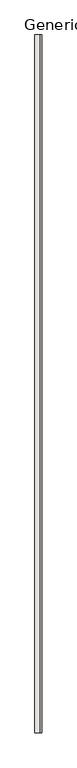
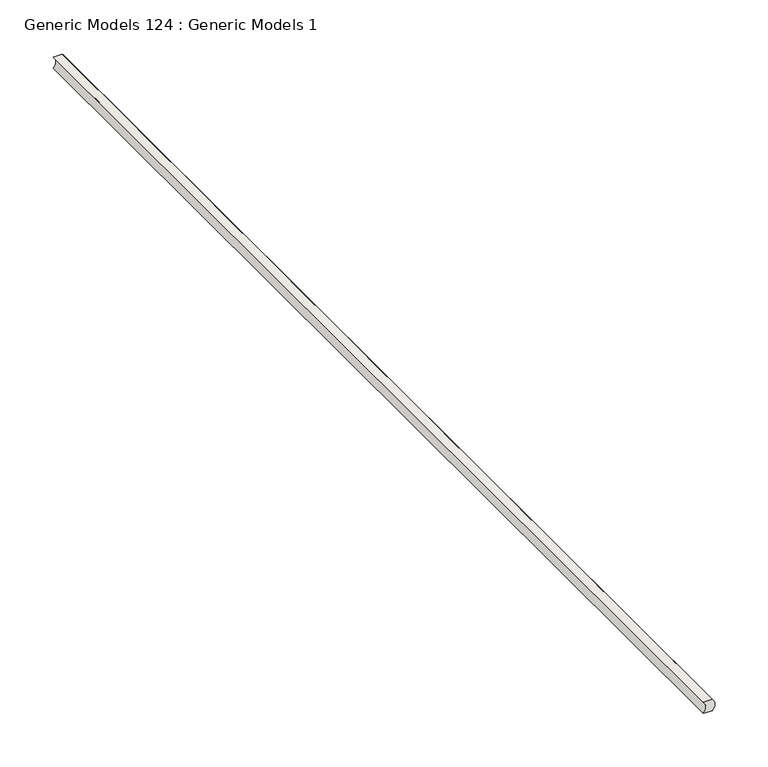
"""IFC4 building model written with IfcOpenShell, lengths in millimetres: wall geometry, Generic Models 124 : Generic Models 1."""

import ifcopenshell
import ifcopenshell.guid

model = None  # the IFC model being written
_history = None  # IfcOwnerHistory: only IFC2X3 demands one
_inside = {}  # id of a spatial element -> (the spatial element, [elements in it])
_under = {}  # id of a project, library or spatial element -> (it, [spatial elements below it])
_declared = {}  # id of a project -> (the project, [libraries it declares])
_typed = {}  # id of a type object -> (the type object, [elements of that type])
_made_of = {}  # id of a material, layer set ... -> (it, [elements and type objects made of it])


def new_model(schema):
    """Start an empty IFC model of exactly this schema.

    Asked for "IFC4X3", IfcOpenShell would pick the latest addendum, in which some entities
    have other attributes; the version numbers below select the first issue.
    IFC2X3 requires an IfcOwnerHistory on every rooted entity: one is made here for all.
    """
    global model, _history
    if schema == "IFC4X3":
        model = ifcopenshell.file(schema_version=(4, 3, 0, 0))
    else:
        model = ifcopenshell.file(schema=schema)
    _inside.clear()
    _under.clear()
    _declared.clear()
    _typed.clear()
    _made_of.clear()
    _history = None
    if model.schema == "IFC2X3":
        org = make("IfcOrganization", Name="unknown")
        user = make(
            "IfcPersonAndOrganization",
            ThePerson=make("IfcPerson", FamilyName="unknown"),
            TheOrganization=org,
        )
        app = make(
            "IfcApplication",
            ApplicationDeveloper=org,
            Version="unknown",
            ApplicationFullName="unknown",
            ApplicationIdentifier="unknown",
        )
        _history = make(
            "IfcOwnerHistory",
            OwningUser=user,
            OwningApplication=app,
            ChangeAction="ADDED",
            CreationDate=0,
        )
    return model


def make(cls, **values):
    """One entity of the class cls with the attributes given. An attribute that is None is left unset."""
    return model.create_entity(
        cls, **{name: value for name, value in values.items() if value is not None}
    )


def rooted(cls, **values):
    """An entity with a GlobalId (a new one), such as an element, a storey or a relation."""
    return make(cls, GlobalId=ifcopenshell.guid.new(), OwnerHistory=_history, **values)


def si_unit(unit_type, name, prefix=None):
    """IfcSIUnit, for example si_unit("LENGTHUNIT", "METRE", prefix="MILLI")."""
    return make("IfcSIUnit", UnitType=unit_type, Prefix=prefix, Name=name)


def assignment(units):
    """IfcUnitAssignment: the units of a project."""
    return None if units is None else make("IfcUnitAssignment", Units=units)


def point(xyz):
    """IfcCartesianPoint."""
    return None if xyz is None else make("IfcCartesianPoint", Coordinates=xyz)


def direction(xyz):
    """IfcDirection."""
    return None if xyz is None else make("IfcDirection", DirectionRatios=xyz)


def frame(location, z_axis=None, x_axis=None):
    """IfcAxis2Placement3D, a coordinate frame: its origin and axes. An axis left out is left unset."""
    return make(
        "IfcAxis2Placement3D",
        Location=point(location),
        Axis=direction(z_axis),
        RefDirection=direction(x_axis),
    )


def frame_2d(location, x_axis=None):
    """IfcAxis2Placement2D, a coordinate frame in the plane: its origin and x axis."""
    return make(
        "IfcAxis2Placement2D", Location=point(location), RefDirection=direction(x_axis)
    )


def origin():
    """The frame at (0, 0, 0) with its axes left unset."""
    return frame((0.0, 0.0, 0.0))


def place(relative_to, where):
    """IfcLocalPlacement: puts the frame where relative to a parent placement (None: the world)."""
    return make(
        "IfcLocalPlacement", PlacementRelTo=relative_to, RelativePlacement=where
    )


def context(
    kind, dimensions, precision=None, world=None, true_north=None, identifier=None
):
    """IfcGeometricRepresentationContext, for example the 3D "Model" context."""
    return make(
        "IfcGeometricRepresentationContext",
        ContextIdentifier=identifier,
        ContextType=kind,
        CoordinateSpaceDimension=dimensions,
        Precision=precision,
        WorldCoordinateSystem=world,
        TrueNorth=true_north,
    )


def project(units=None, contexts=None):
    """IfcProject with its units and contexts."""
    return rooted(
        "IfcProject",
        Name="project",
        RepresentationContexts=contexts,
        UnitsInContext=assignment(units),
    )


def spatial(cls, under=None, at=None, **own):
    """A site, building, storey or space (cls), placed at a placement, below another one or the project."""
    s = rooted(cls, ObjectPlacement=at, **own)
    if under is not None:
        _under.setdefault(under.id(), (under, []))[1].append(s)
    return s


def polyline(points):
    """IfcPolyline through the points."""
    return make("IfcPolyline", Points=[point(p) for p in points])


def circle_curve(where, radius):
    """IfcCircle in the frame where."""
    return make("IfcCircle", Position=where, Radius=radius)


def trimmed(basis, trim1, trim2, sense, master):
    """IfcTrimmedCurve: the piece of a basis curve between two trims."""
    return make(
        "IfcTrimmedCurve",
        BasisCurve=basis,
        Trim1=trim1,
        Trim2=trim2,
        SenseAgreement=sense,
        MasterRepresentation=master,
    )


def segment(curve, same_sense, transition):
    """IfcCompositeCurveSegment."""
    return make(
        "IfcCompositeCurveSegment",
        Transition=transition,
        SameSense=same_sense,
        ParentCurve=curve,
    )


def composite_curve(segments, self_intersect=None):
    """IfcCompositeCurve: segments joined end to end."""
    return make("IfcCompositeCurve", Segments=segments, SelfIntersect=self_intersect)


def outline(outer, holes=None, kind="AREA"):
    """IfcArbitraryClosedProfileDef: a profile drawn as a closed curve; with holes, ...WithVoids."""
    if holes is None:
        return make("IfcArbitraryClosedProfileDef", ProfileType=kind, OuterCurve=outer)
    return make(
        "IfcArbitraryProfileDefWithVoids",
        ProfileType=kind,
        OuterCurve=outer,
        InnerCurves=holes,
    )


def extrude(swept, where, along, depth):
    """IfcExtrudedAreaSolid: the profile swept, set in the frame where, extruded along a direction by depth."""
    return make(
        "IfcExtrudedAreaSolid",
        SweptArea=swept,
        Position=where,
        ExtrudedDirection=direction(along),
        Depth=depth,
    )


def shape(context_of_items, identifier, shape_type, items):
    """IfcShapeRepresentation: the items that make up one representation, for example the "Body"."""
    return make(
        "IfcShapeRepresentation",
        ContextOfItems=context_of_items,
        RepresentationIdentifier=identifier,
        RepresentationType=shape_type,
        Items=items,
    )


def source(mapping_origin, context_of_items, identifier, shape_type, items):
    """IfcRepresentationMap: a shape defined once, which mapped items show again and again."""
    return make(
        "IfcRepresentationMap",
        MappingOrigin=mapping_origin,
        MappedRepresentation=shape(context_of_items, identifier, shape_type, items),
    )


def transform(
    local_origin,
    x_axis=None,
    y_axis=None,
    z_axis=None,
    scale=None,
    scale2=None,
    scale3=None,
    uniform=True,
):
    """IfcCartesianTransformationOperator3D, or its non-uniform kind. x_axis, y_axis, z_axis: its Axis1, 2, 3."""
    if uniform:
        return make(
            "IfcCartesianTransformationOperator3D",
            Axis1=direction(x_axis),
            Axis2=direction(y_axis),
            LocalOrigin=point(local_origin),
            Scale=scale,
            Axis3=direction(z_axis),
        )
    return make(
        "IfcCartesianTransformationOperator3DnonUniform",
        Axis1=direction(x_axis),
        Axis2=direction(y_axis),
        LocalOrigin=point(local_origin),
        Scale=scale,
        Axis3=direction(z_axis),
        Scale2=scale2,
        Scale3=scale3,
    )


def mapped(mapping_source, mapping_target):
    """IfcMappedItem: shows the shape of a source again, moved by a transform."""
    return make(
        "IfcMappedItem", MappingSource=mapping_source, MappingTarget=mapping_target
    )


def made_of(thing, what):
    """Note that an element or type object is made of a material, layer set ...; save() writes the relation."""
    if what is not None:
        _made_of.setdefault(what.id(), (what, []))[1].append(thing)
    return thing


def element(
    cls,
    number,
    at=None,
    inside=None,
    cuts=None,
    type_object=None,
    material=None,
    context=None,
    identifier="Body",
    shape_type=None,
    held_by="IfcProductDefinitionShape",
    body=None,
    shapes=None,
    **own,
):
    """One element of the class cls, such as IfcWall. Its Tag is "e" and its number.

    at: its placement. inside: the storey or other place that contains it. cuts: it is an
    opening in that element (IfcRelVoidsElement). A single representation is given by context,
    identifier, shape_type and body (its items); several are given by shapes. held_by: the class
    of the entity that holds the representations. save() writes the other relations.
    """
    e = rooted(cls, Tag="e%d" % number, ObjectPlacement=at, **own)
    if body is not None:
        shapes = [shape(context, identifier, shape_type, body)]
    if shapes is not None:
        e.Representation = make(held_by, Representations=shapes)
    if inside is not None:
        _inside.setdefault(inside.id(), (inside, []))[1].append(e)
    if cuts is not None:
        rooted(
            "IfcRelVoidsElement", RelatingBuildingElement=cuts, RelatedOpeningElement=e
        )
    if type_object is not None:
        _typed.setdefault(type_object.id(), (type_object, []))[1].append(e)
    return made_of(e, material)


def aggregate(whole, parts):
    """IfcRelAggregates: a whole, such as a stair, and the parts it consists of."""
    return rooted("IfcRelAggregates", RelatingObject=whole, RelatedObjects=parts)


def save(model, path):
    """Write the relations noted so far, then the file.

    IfcRelAggregates (storeys below a building ...), IfcRelContainedInSpatialStructure (elements
    in a storey), IfcRelDefinesByType, IfcRelAssociatesMaterial and IfcRelDeclares: one each for
    every whole, place, type object, material and project.
    """
    for whole, parts in _under.values():
        aggregate(whole, parts)
    for where, things in _inside.values():
        rooted(
            "IfcRelContainedInSpatialStructure",
            RelatedElements=things,
            RelatingStructure=where,
        )
    for kind, things in _typed.values():
        rooted("IfcRelDefinesByType", RelatedObjects=things, RelatingType=kind)
    for what, things in _made_of.values():
        rooted("IfcRelAssociatesMaterial", RelatedObjects=things, RelatingMaterial=what)
    for by, libraries in _declared.values():
        rooted("IfcRelDeclares", RelatingContext=by, RelatedDefinitions=libraries)
    model.write(path)


def generic_models_124_generic_models_1_37c4acb5(model_context):
    return source(origin(), model_context, "Body", "SweptSolid", [
        extrude(outline(composite_curve([segment(polyline([(1809.9484375, 50900.0125), (1809.9484375, 50909.5375)]), True, "CONTINUOUS"), segment(trimmed(circle_curve(frame_2d((1816.2984375, 50903.708019)), 8.620055), [point((1809.9484375, 50909.5375))], [point((1822.6484375, 50909.5375))], False, "CARTESIAN"), True, "CONTINUOUS"), segment(polyline([(1822.6484375, 50909.5375), (1822.6484375, 50900.0125)]), True, "CONTINUOUS"), segment(trimmed(circle_curve(frame_2d((1816.2984375, 50894.183019)), 8.620055), [point((1822.6484375, 50900.0125))], [point((1809.9484375, 50900.0125))], True, "CARTESIAN"), True, "CONTINUOUS")], self_intersect=False)), frame((0.0, 0.0, 0.0), z_axis=(0.0, 1.0, 0.0), x_axis=(0.0, 0.0, 1.0)), (0.0, 0.0, 1.0), 1219.2),
    ])


if __name__ == "__main__":
    model = new_model("IFC4")
    model_context = context("Model", 3, world=origin())
    ifc_project = project(units=[si_unit("LENGTHUNIT", "METRE", prefix="MILLI")], contexts=[model_context])
    site = spatial("IfcSite", under=ifc_project)
    building = spatial("IfcBuilding", under=site)
    placement = place(None, origin())
    generic_models_124_generic_models_1_shape = generic_models_124_generic_models_1_37c4acb5(model_context)
    element("IfcWall", 1, ObjectType="Generic Models 124 : Generic Models 1", at=placement, inside=building, context=model_context, shape_type="MappedRepresentation", body=[
        mapped(generic_models_124_generic_models_1_shape, transform((0.0, 0.0, 0.0), x_axis=(1.0, 0.0, 0.0), y_axis=(0.0, 1.0, 0.0), z_axis=(0.0, 0.0, 1.0))),
    ])
    save(model, "model.ifc")

# Revit data of these elements
# Element 1 (IfcWall, "Generic Models 124 : Generic Models 1")
#   Materials on its faces: "SEALANT (W/ BACKER ROD IF NECESSARY)"
# Materials
#   "SEALANT (W/ BACKER ROD IF NECESSARY)": class "Unassigned", colour RGB 120 120 120, transparency 0, Cost = 0
